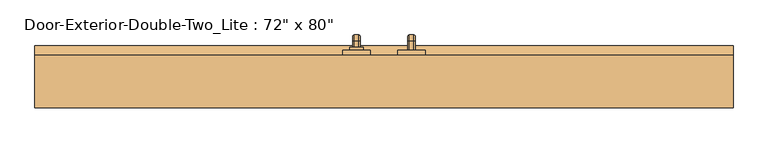
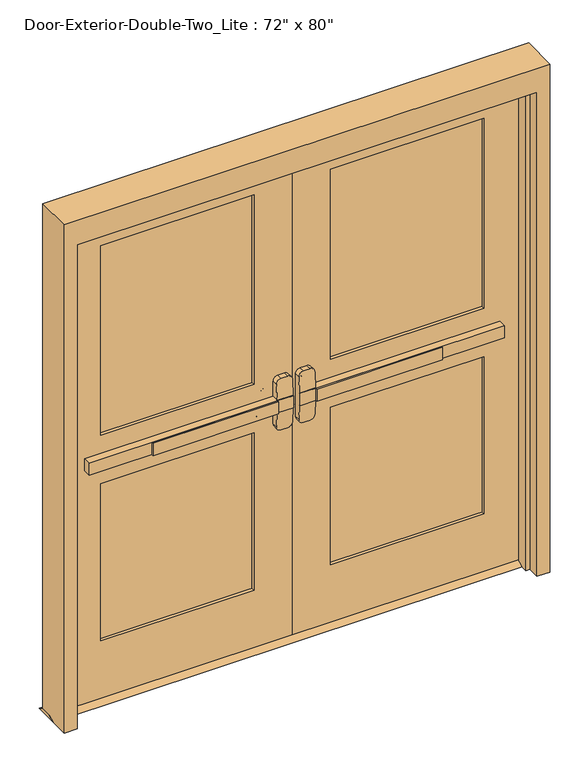
"""IFC4 building model written with IfcOpenShell, lengths in millimetres: door geometry."""

from ifc_helpers import new_model, si_unit, point, frame, frame_2d, origin, place, context, project, spatial, polyline, circle_curve, ellipse_curve, trimmed, segment, composite_curve, outline, extrude, faceted_brep, source, transform, mapped, element, save
from ifc_brep_helpers import plane_surface, cylinder_surface, revolved_surface, advanced_brep


def door_7ac9a1dc(model_context):
    return source(origin(), model_context, "Body", "SolidModel", [
        extrude(outline(polyline([(-575.7333333, -3.175), (-575.7333333, 3.175), (-76.2, 3.175), (-76.2, -3.175), (-575.7333333, -3.175)])), frame((0.0, 0.0, 990.6), z_axis=(0.0, 0.0, 1.0), x_axis=(1.0, 0.0, 0.0)), (0.0, 0.0, 1.0), 50.8),
        advanced_brep(
        [(-12.7, 3.175, 1041.4), (-76.2, 3.175, 1041.4), (-825.5, 3.175, 1041.4), (-825.5, 3.175, 990.6), (-76.2, 3.175, 990.6), (-12.7, 3.175, 990.6), (-825.5, 34.925, 1041.4), (-76.2, 34.925, 1041.4), (-76.2, 34.925, 1104.9), (-57.15, 34.925, 1123.95), (-31.75, 34.925, 1123.95), (-12.7, 34.925, 1104.9), (-12.7, 34.925, 927.1), (-31.75, 34.925, 908.05), (-57.15, 34.925, 908.05), (-76.2, 34.925, 927.1), (-76.2, 34.925, 990.6), (-825.5, 34.925, 990.6), (-12.7, 6.3502467, 1041.4), (-76.2, 6.3502467, 1041.4), (-12.7, 6.3502467, 990.6), (-12.7, 11.3604269, 927.1), (-12.7, 11.3604269, 1104.9), (-76.2, 6.3502467, 990.6), (-76.2, 11.3604269, 1104.9), (-76.2, 11.3604269, 927.1), (-57.15, 12.863481, 1123.95), (-31.75, 12.863481, 1123.95), (-31.75, 12.863481, 908.05), (-57.15, 12.863481, 908.05)],
        [
            (0, 1),
            (1, 2),
            (2, 3),
            (3, 4),
            (4, 5),
            (5, 0),
            (6, 7),
            (7, 8),
            (8, 9, circle_curve(frame((-57.15, 34.925, 1104.9), z_axis=(0.0, 1.0, 0.0), x_axis=(-1.0, 0.0, 0.0)), 19.05)),
            (9, 10),
            (10, 11, circle_curve(frame((-31.75, 34.925, 1104.9), z_axis=(0.0, 1.0, 0.0), x_axis=(-1.0, 0.0, 0.0)), 19.05)),
            (11, 12),
            (12, 13, circle_curve(frame((-31.75, 34.925, 927.1), z_axis=(0.0, 1.0, 0.0), x_axis=(-1.0, 0.0, 0.0)), 19.05)),
            (13, 14),
            (14, 15, circle_curve(frame((-57.15, 34.925, 927.1), z_axis=(0.0, 1.0, 0.0), x_axis=(-1.0, 0.0, 0.0)), 19.05)),
            (15, 16),
            (16, 17),
            (17, 6),
            (0, 18),
            (18, 19),
            (19, 7),
            (6, 2),
            (5, 20),
            (20, 21),
            (21, 12),
            (11, 22),
            (22, 18),
            (16, 23),
            (23, 20),
            (3, 17),
            (19, 24),
            (24, 8),
            (15, 25),
            (25, 23),
            (9, 26),
            (26, 27),
            (27, 10),
            (13, 28),
            (28, 29),
            (29, 14),
            (29, 25, ellipse_curve(frame((-57.15, 11.3604269, 927.1), z_axis=(0.0, 0.9969018152893365, 0.07865602756830282), x_axis=(0.0, -0.07865602756830208, 0.9969018152893365)), 19.1092038, 19.05)),
            (24, 26, ellipse_curve(frame((-57.15, 11.3604269, 1104.9), z_axis=(0.0, 0.9969018152893376, -0.07865602756828934), x_axis=(0.0, -0.078656027568288, -0.9969018152893377)), 19.1092038, 19.05)),
            (27, 22, ellipse_curve(frame((-31.75, 11.3604269, 1104.9), z_axis=(0.0, 0.9969018152893376, -0.07865602756828934), x_axis=(0.0, -0.078656027568288, -0.9969018152893377)), 19.1092038, 19.05)),
            (21, 28, ellipse_curve(frame((-31.75, 11.3604269, 927.1), z_axis=(0.0, 0.9969018152893365, 0.07865602756830282), x_axis=(0.0, -0.07865602756830208, 0.9969018152893365)), 19.1092038, 19.05)),
        ],
        [
            plane_surface(frame((-12.7, 3.175, 1041.4), z_axis=(0.0, -1.0, 0.0), x_axis=(1.0, 0.0, 0.0))),
            plane_surface(frame((-12.7, 34.925, 1041.4), z_axis=(0.0, 1.0, 0.0), x_axis=(-1.0, 0.0, 0.0))),
            plane_surface(frame((-825.5, 3.175, 1041.4), z_axis=(0.0, 0.0, 1.0), x_axis=(0.0, 1.0, 0.0))),
            plane_surface(frame((-12.7, 3.175, 1041.4), z_axis=(1.0, 0.0, 0.0), x_axis=(0.0, 1.0, 0.0))),
            plane_surface(frame((-12.7, 3.175, 990.6), z_axis=(0.0, 0.0, -1.0), x_axis=(0.0, 1.0, 0.0))),
            plane_surface(frame((-825.5, 3.175, 990.6), z_axis=(-1.0, 0.0, 0.0), x_axis=(0.0, 1.0, 0.0))),
            plane_surface(frame((-76.2, 6.3502467, 927.1), z_axis=(-1.0, 0.0, 0.0), x_axis=(0.0, 1.0, 0.0))),
            plane_surface(frame((-57.15, 6.3502467, 1123.95), z_axis=(0.0, 0.0, 1.0), x_axis=(0.0, 1.0, 0.0))),
            plane_surface(frame((-31.75, 6.3502467, 908.05), z_axis=(0.0, 0.0, -1.0), x_axis=(0.0, 1.0, 0.0))),
            cylinder_surface(frame((-57.15, 34.925, 927.1), z_axis=(0.0, -1.0, 0.0), x_axis=(-1.0, 0.0, 0.0)), 19.05),
            cylinder_surface(frame((-57.15, 34.925, 1104.9), z_axis=(0.0, -1.0, 0.0), x_axis=(-1.0, 0.0, 0.0)), 19.05),
            cylinder_surface(frame((-31.75, 34.925, 1104.9), z_axis=(0.0, -1.0, 0.0), x_axis=(-1.0, 0.0, 0.0)), 19.05),
            cylinder_surface(frame((-31.75, 34.925, 927.1), z_axis=(0.0, -1.0, 0.0), x_axis=(-1.0, 0.0, 0.0)), 19.05),
            plane_surface(frame((-76.2, 6.3502467, 1041.4), z_axis=(0.0, -0.9969018152893376, 0.07865602756828934), x_axis=(1.0, 0.0, 0.0))),
            plane_surface(frame((-76.2, 12.863481, 908.05), z_axis=(0.0, -0.9969018152893365, -0.07865602756830282), x_axis=(1.0, 0.0, 0.0))),
        ],
        [
            (0, [[1, 2, 3, 4, 5, 6]]),
            (1, [[7, 8, 9, 10, 11, 12, 13, 14, 15, 16, 17, 18]]),
            (2, [[-2, -1, 19, 20, 21, -7, 22]]),
            (3, [[23, 24, 25, -12, 26, 27, -19, -6]]),
            (4, [[-17, 28, 29, -23, -5, -4, 30]]),
            (5, [[-22, -18, -30, -3]]),
            (6, [[-21, 31, 32, -8]]),
            (6, [[33, 34, -28, -16]]),
            (7, [[35, 36, 37, -10]]),
            (8, [[38, 39, 40, -14]]),
            (9, [[-40, 41, -33, -15]]),
            (10, [[-32, 42, -35, -9]]),
            (11, [[-37, 43, -26, -11]]),
            (12, [[-25, 44, -38, -13]]),
            (13, [[-27, -43, -36, -42, -31, -20]]),
            (14, [[-29, -34, -41, -39, -44, -24]]),
        ],
    ),
        extrude(outline(polyline([(79.375, 12.7), (104.775, 0.0), (9.525, 0.0), (34.925, 12.7), (79.375, 12.7)])), frame((-965.2, 0.0, 0.0), z_axis=(1.0, 0.0, 0.0), x_axis=(0.0, 1.0, 0.0)), (0.0, 0.0, 1.0), 1930.4),
        extrude(outline(polyline([(575.7333333, -3.175), (76.2, -3.175), (76.2, 3.175), (575.7333333, 3.175), (575.7333333, -3.175)])), frame((0.0, 0.0, 990.6), z_axis=(0.0, 0.0, 1.0), x_axis=(1.0, 0.0, 0.0)), (0.0, 0.0, 1.0), 50.8),
        advanced_brep(
        [(12.7, 3.175, 1041.4), (12.7, 3.175, 990.6), (76.2, 3.175, 990.6), (825.5, 3.175, 990.6), (825.5, 3.175, 1041.4), (76.2, 3.175, 1041.4), (825.5, 34.925, 1041.4), (825.5, 34.925, 990.6), (76.2, 34.925, 990.6), (76.2, 34.925, 927.1), (57.15, 34.925, 908.05), (31.75, 34.925, 908.05), (12.7, 34.925, 927.1), (12.7, 34.925, 1104.9), (31.75, 34.925, 1123.95), (57.15, 34.925, 1123.95), (76.2, 34.925, 1104.9), (76.2, 34.925, 1041.4), (76.2, 6.3502467, 1041.4), (12.7, 6.3502467, 1041.4), (12.7, 11.3604269, 1104.9), (12.7, 11.3604269, 927.1), (12.7, 6.3502467, 990.6), (76.2, 6.3502467, 990.6), (76.2, 11.3604269, 927.1), (76.2, 11.3604269, 1104.9), (31.75, 12.863481, 1123.95), (57.15, 12.863481, 1123.95), (57.15, 12.863481, 908.05), (31.75, 12.863481, 908.05)],
        [
            (0, 1),
            (1, 2),
            (2, 3),
            (3, 4),
            (4, 5),
            (5, 0),
            (6, 7),
            (7, 8),
            (8, 9),
            (9, 10, circle_curve(frame((57.15, 34.925, 927.1), z_axis=(0.0, 1.0, 0.0), x_axis=(1.0, 0.0, 0.0)), 19.05)),
            (10, 11),
            (11, 12, circle_curve(frame((31.75, 34.925, 927.1), z_axis=(0.0, 1.0, 0.0), x_axis=(1.0, 0.0, 0.0)), 19.05)),
            (12, 13),
            (13, 14, circle_curve(frame((31.75, 34.925, 1104.9), z_axis=(0.0, 1.0, 0.0), x_axis=(1.0, 0.0, 0.0)), 19.05)),
            (14, 15),
            (15, 16, circle_curve(frame((57.15, 34.925, 1104.9), z_axis=(0.0, 1.0, 0.0), x_axis=(1.0, 0.0, 0.0)), 19.05)),
            (16, 17),
            (17, 6),
            (4, 6),
            (17, 18),
            (18, 19),
            (19, 0),
            (19, 20),
            (20, 13),
            (12, 21),
            (21, 22),
            (22, 1),
            (7, 3),
            (22, 23),
            (23, 8),
            (23, 24),
            (24, 9),
            (16, 25),
            (25, 18),
            (14, 26),
            (26, 27),
            (27, 15),
            (10, 28),
            (28, 29),
            (29, 11),
            (24, 28, ellipse_curve(frame((57.15, 11.3604269, 927.1), z_axis=(0.0, 0.9969018152893365, 0.07865602756830282), x_axis=(0.0, -0.07865602756830208, 0.9969018152893365)), 19.1092038, 19.05)),
            (27, 25, ellipse_curve(frame((57.15, 11.3604269, 1104.9), z_axis=(0.0, 0.9969018152893376, -0.07865602756828934), x_axis=(0.0, -0.078656027568288, -0.9969018152893377)), 19.1092038, 19.05)),
            (20, 26, ellipse_curve(frame((31.75, 11.3604269, 1104.9), z_axis=(0.0, 0.9969018152893376, -0.07865602756828934), x_axis=(0.0, -0.078656027568288, -0.9969018152893377)), 19.1092038, 19.05)),
            (29, 21, ellipse_curve(frame((31.75, 11.3604269, 927.1), z_axis=(0.0, 0.9969018152893365, 0.07865602756830282), x_axis=(0.0, -0.07865602756830208, 0.9969018152893365)), 19.1092038, 19.05)),
        ],
        [
            plane_surface(frame((12.7, 3.175, 1041.4), z_axis=(0.0, -1.0, 0.0), x_axis=(-1.0, 0.0, 0.0))),
            plane_surface(frame((12.7, 34.925, 1041.4), z_axis=(0.0, 1.0, 0.0), x_axis=(1.0, 0.0, 0.0))),
            plane_surface(frame((825.5, 3.175, 1041.4), z_axis=(0.0, 0.0, 1.0), x_axis=(0.0, 1.0, 0.0))),
            plane_surface(frame((12.7, 3.175, 1041.4), z_axis=(-1.0, 0.0, 0.0), x_axis=(0.0, 1.0, 0.0))),
            plane_surface(frame((12.7, 3.175, 990.6), z_axis=(0.0, 0.0, -1.0), x_axis=(0.0, 1.0, 0.0))),
            plane_surface(frame((825.5, 3.175, 990.6), z_axis=(1.0, 0.0, 0.0), x_axis=(0.0, 1.0, 0.0))),
            plane_surface(frame((76.2, 6.3502467, 927.1), z_axis=(1.0, 0.0, 0.0), x_axis=(0.0, 1.0, 0.0))),
            plane_surface(frame((57.15, 6.3502467, 1123.95), z_axis=(0.0, 0.0, 1.0), x_axis=(0.0, 1.0, 0.0))),
            plane_surface(frame((31.75, 6.3502467, 908.05), z_axis=(0.0, 0.0, -1.0), x_axis=(0.0, 1.0, 0.0))),
            cylinder_surface(frame((57.15, 34.925, 927.1), z_axis=(0.0, -1.0, 0.0), x_axis=(1.0, 0.0, 0.0)), 19.05),
            cylinder_surface(frame((57.15, 34.925, 1104.9), z_axis=(0.0, -1.0, 0.0), x_axis=(1.0, 0.0, 0.0)), 19.05),
            cylinder_surface(frame((31.75, 34.925, 1104.9), z_axis=(0.0, -1.0, 0.0), x_axis=(1.0, 0.0, 0.0)), 19.05),
            cylinder_surface(frame((31.75, 34.925, 927.1), z_axis=(0.0, -1.0, 0.0), x_axis=(1.0, 0.0, 0.0)), 19.05),
            plane_surface(frame((76.2, 6.3502467, 1041.4), z_axis=(0.0, -0.9969018152893376, 0.07865602756828934), x_axis=(-1.0, 0.0, 0.0))),
            plane_surface(frame((76.2, 12.863481, 908.05), z_axis=(0.0, -0.9969018152893365, -0.07865602756830282), x_axis=(-1.0, 0.0, 0.0))),
        ],
        [
            (0, [[1, 2, 3, 4, 5, 6]]),
            (1, [[7, 8, 9, 10, 11, 12, 13, 14, 15, 16, 17, 18]]),
            (2, [[19, -18, 20, 21, 22, -6, -5]]),
            (3, [[-1, -22, 23, 24, -13, 25, 26, 27]]),
            (4, [[28, -3, -2, -27, 29, 30, -8]]),
            (5, [[-4, -28, -7, -19]]),
            (6, [[-9, -30, 31, 32]]),
            (6, [[-17, 33, 34, -20]]),
            (7, [[-15, 35, 36, 37]]),
            (8, [[-11, 38, 39, 40]]),
            (9, [[-10, -32, 41, -38]]),
            (10, [[-16, -37, 42, -33]]),
            (11, [[-14, -24, 43, -35]]),
            (12, [[-12, -40, 44, -25]]),
            (13, [[-21, -34, -42, -36, -43, -23]]),
            (14, [[-26, -44, -39, -41, -31, -29]]),
        ],
    ),
        advanced_brep(
        [(66.2, 92.075, 1017.190625), (66.2, 92.075, 1014.809375), (69.771875, 92.075, 1011.2375), (82.6284594, 92.075, 1011.2375), (86.2, 92.075, 1014.8090406), (86.2, 92.075, 1017.190625), (82.628125, 92.075, 1020.7625), (69.771875, 92.075, 1020.7625), (66.2, 92.075, 887.809375), (69.771875, 92.075, 884.2375), (82.628125, 92.075, 884.2375), (86.2, 92.075, 887.809375), (86.2, 92.075, 890.1909594), (82.6284594, 92.075, 893.7625), (69.771875, 92.075, 893.7625), (66.2, 92.075, 890.190625), (66.2, 117.475, 1017.190625), (66.2, 131.365625, 1003.3), (66.2, 131.365625, 901.7), (66.2, 117.475, 887.809375), (66.2, 117.475, 890.190625), (66.2, 128.984375, 901.7), (66.2, 128.984375, 1003.3), (66.2, 117.475, 1014.809375), (69.771875, 117.475, 1011.2375), (82.6284594, 117.475, 1011.2375), (86.2, 117.475, 1014.8090406), (86.2, 128.9840406, 1003.3), (86.2, 128.9840406, 901.7), (86.2, 117.475, 890.1909594), (86.2, 117.475, 887.809375), (86.2, 131.365625, 901.7), (86.2, 131.365625, 1003.3), (86.2, 117.475, 1017.190625), (82.628125, 117.475, 1020.7625), (69.771875, 117.475, 1020.7625), (69.771875, 125.4125, 1003.3), (82.6284594, 125.4125, 1003.3), (82.628125, 134.9375, 1003.3), (69.771875, 134.9375, 1003.3), (69.771875, 125.4125, 901.7), (82.6284594, 125.4125, 901.7), (82.628125, 134.9375, 901.7), (69.771875, 134.9375, 901.7), (69.771875, 117.475, 893.7625), (82.6284594, 117.475, 893.7625), (82.628125, 117.475, 884.2375), (69.771875, 117.475, 884.2375)],
        [
            (0, 1),
            (1, 2, circle_curve(frame((69.771875, 92.075, 1014.809375), z_axis=(0.0, -1.0, 0.0), x_axis=(0.0, 0.0, 1.0)), 3.571875)),
            (2, 3),
            (3, 4, circle_curve(frame((82.6284594, 92.075, 1014.8090406), z_axis=(0.0, -1.0, 0.0), x_axis=(0.0, 0.0, 1.0)), 3.5715406)),
            (4, 5),
            (5, 6, circle_curve(frame((82.628125, 92.075, 1017.190625), z_axis=(0.0, -1.0, 0.0), x_axis=(0.0, 0.0, 1.0)), 3.571875)),
            (6, 7),
            (7, 0, circle_curve(frame((69.771875, 92.075, 1017.190625), z_axis=(0.0, -1.0, 0.0), x_axis=(0.0, 0.0, 1.0)), 3.571875)),
            (8, 9, circle_curve(frame((69.771875, 92.075, 887.809375), z_axis=(0.0, -1.0, 0.0), x_axis=(0.0, 0.0, -1.0)), 3.571875)),
            (9, 10),
            (10, 11, circle_curve(frame((82.628125, 92.075, 887.809375), z_axis=(0.0, -1.0, 0.0), x_axis=(0.0, 0.0, -1.0)), 3.571875)),
            (11, 12),
            (12, 13, circle_curve(frame((82.6284594, 92.075, 890.1909594), z_axis=(0.0, -1.0, 0.0), x_axis=(0.0, 0.0, -1.0)), 3.5715406)),
            (13, 14),
            (14, 15, circle_curve(frame((69.771875, 92.075, 890.190625), z_axis=(0.0, -1.0, 0.0), x_axis=(0.0, 0.0, -1.0)), 3.571875)),
            (15, 8),
            (0, 16),
            (16, 17, circle_curve(frame((66.2, 117.475, 1003.3), z_axis=(-1.0, 0.0, 0.0), x_axis=(0.0, 0.0, 1.0)), 13.890625)),
            (17, 18),
            (18, 19, circle_curve(frame((66.2, 117.475, 901.7), z_axis=(-1.0, 0.0, 0.0), x_axis=(0.0, 1.0, 0.0)), 13.890625)),
            (19, 8),
            (15, 20),
            (20, 21, circle_curve(frame((66.2, 117.475, 901.7), z_axis=(1.0, 0.0, 0.0), x_axis=(0.0, 1.0, 0.0)), 11.509375)),
            (21, 22),
            (22, 23, circle_curve(frame((66.2, 117.475, 1003.3), z_axis=(1.0, 0.0, 0.0), x_axis=(0.0, 0.0, 1.0)), 11.509375)),
            (23, 1),
            (23, 24, circle_curve(frame((69.771875, 117.475, 1014.809375), z_axis=(0.0, -1.0, 0.0), x_axis=(0.0, 0.0, 1.0)), 3.571875)),
            (24, 2),
            (24, 25),
            (25, 3),
            (25, 26, circle_curve(frame((82.6284594, 117.475, 1014.8090406), z_axis=(0.0, -1.0, 0.0), x_axis=(0.0, 0.0, 1.0)), 3.5715406)),
            (26, 4),
            (26, 27, circle_curve(frame((86.2, 117.475, 1003.3), z_axis=(-1.0, 0.0, 0.0), x_axis=(0.0, 0.0, 1.0)), 11.5090406)),
            (27, 28),
            (28, 29, circle_curve(frame((86.2, 117.475, 901.7), z_axis=(-1.0, 0.0, 0.0), x_axis=(0.0, 1.0, 0.0)), 11.5090406)),
            (29, 12),
            (11, 30),
            (30, 31, circle_curve(frame((86.2, 117.475, 901.7), z_axis=(1.0, 0.0, 0.0), x_axis=(0.0, 1.0, 0.0)), 13.890625)),
            (31, 32),
            (32, 33, circle_curve(frame((86.2, 117.475, 1003.3), z_axis=(1.0, 0.0, 0.0), x_axis=(0.0, 0.0, 1.0)), 13.890625)),
            (33, 5),
            (33, 34, circle_curve(frame((82.628125, 117.475, 1017.190625), z_axis=(0.0, -1.0, 0.0), x_axis=(0.0, 0.0, 1.0)), 3.571875)),
            (34, 6),
            (34, 35),
            (35, 7),
            (35, 16, circle_curve(frame((69.771875, 117.475, 1017.190625), z_axis=(0.0, -1.0, 0.0), x_axis=(0.0, 0.0, 1.0)), 3.571875)),
            (36, 24, circle_curve(frame((69.771875, 117.475, 1003.3), z_axis=(1.0, 0.0, 0.0), x_axis=(0.0, 0.0, 1.0)), 7.9375)),
            (22, 36, circle_curve(frame((69.771875, 128.984375, 1003.3), z_axis=(0.0, 0.0, 1.0), x_axis=(0.0, 1.0, 0.0)), 3.571875)),
            (37, 25, circle_curve(frame((82.6284594, 117.475, 1003.3), z_axis=(1.0, 0.0, 0.0), x_axis=(0.0, 0.0, 1.0)), 7.9375)),
            (36, 37),
            (37, 27, circle_curve(frame((82.6284594, 128.9840406, 1003.3), z_axis=(0.0, 0.0, 1.0), x_axis=(0.0, 1.0, 0.0)), 3.5715406)),
            (38, 34, circle_curve(frame((82.628125, 117.475, 1003.3), z_axis=(1.0, 0.0, 0.0), x_axis=(0.0, 0.0, 1.0)), 17.4625)),
            (32, 38, circle_curve(frame((82.628125, 131.365625, 1003.3), z_axis=(0.0, 0.0, 1.0), x_axis=(0.0, 1.0, 0.0)), 3.571875)),
            (39, 35, circle_curve(frame((69.771875, 117.475, 1003.3), z_axis=(1.0, 0.0, 0.0), x_axis=(0.0, 0.0, 1.0)), 17.4625)),
            (38, 39),
            (39, 17, circle_curve(frame((69.771875, 131.365625, 1003.3), z_axis=(0.0, 0.0, 1.0), x_axis=(0.0, 1.0, 0.0)), 3.571875)),
            (21, 40, circle_curve(frame((69.771875, 128.984375, 901.7), z_axis=(0.0, 0.0, 1.0), x_axis=(0.0, 1.0, 0.0)), 3.571875)),
            (40, 36),
            (40, 41),
            (41, 37),
            (41, 28, circle_curve(frame((82.6284594, 128.9840406, 901.7), z_axis=(0.0, 0.0, 1.0), x_axis=(0.0, 1.0, 0.0)), 3.5715406)),
            (31, 42, circle_curve(frame((82.628125, 131.365625, 901.7), z_axis=(0.0, 0.0, 1.0), x_axis=(0.0, 1.0, 0.0)), 3.571875)),
            (42, 38),
            (42, 43),
            (43, 39),
            (43, 18, circle_curve(frame((69.771875, 131.365625, 901.7), z_axis=(0.0, 0.0, 1.0), x_axis=(0.0, 1.0, 0.0)), 3.571875)),
            (44, 40, circle_curve(frame((69.771875, 117.475, 901.7), z_axis=(1.0, 0.0, 0.0), x_axis=(0.0, 1.0, 0.0)), 7.9375)),
            (20, 44, circle_curve(frame((69.771875, 117.475, 890.190625), z_axis=(0.0, 1.0, 0.0), x_axis=(0.0, 0.0, -1.0)), 3.571875)),
            (45, 41, circle_curve(frame((82.6284594, 117.475, 901.7), z_axis=(1.0, 0.0, 0.0), x_axis=(0.0, 1.0, 0.0)), 7.9375)),
            (44, 45),
            (45, 29, circle_curve(frame((82.6284594, 117.475, 890.1909594), z_axis=(0.0, 1.0, 0.0), x_axis=(0.0, 0.0, -1.0)), 3.5715406)),
            (46, 42, circle_curve(frame((82.628125, 117.475, 901.7), z_axis=(1.0, 0.0, 0.0), x_axis=(0.0, 1.0, 0.0)), 17.4625)),
            (30, 46, circle_curve(frame((82.628125, 117.475, 887.809375), z_axis=(0.0, 1.0, 0.0), x_axis=(0.0, 0.0, -1.0)), 3.571875)),
            (47, 43, circle_curve(frame((69.771875, 117.475, 901.7), z_axis=(1.0, 0.0, 0.0), x_axis=(0.0, 1.0, 0.0)), 17.4625)),
            (46, 47),
            (47, 19, circle_curve(frame((69.771875, 117.475, 887.809375), z_axis=(0.0, 1.0, 0.0), x_axis=(0.0, 0.0, -1.0)), 3.571875)),
            (14, 44),
            (13, 45),
            (10, 46),
            (9, 47),
        ],
        [
            plane_surface(frame((76.2, 92.075, 1016.0), z_axis=(0.0, -1.0, 0.0), x_axis=(1.0, 0.0, 0.0))),
            plane_surface(frame((76.2, 92.075, 889.0), z_axis=(0.0, -1.0, 0.0), x_axis=(1.0, 0.0, 0.0))),
            plane_surface(frame((66.2, 92.075, 1017.190625), z_axis=(-1.0, 0.0, 0.0), x_axis=(0.0, 1.0, 0.0))),
            cylinder_surface(frame((69.771875, 92.075, 1014.809375), z_axis=(0.0, -1.0, 0.0), x_axis=(0.0, 0.0, 1.0)), 3.571875),
            plane_surface(frame((69.771875, 92.075, 1011.2375), z_axis=(0.0, 0.0, -1.0), x_axis=(0.0, 1.0, 0.0))),
            cylinder_surface(frame((82.6284594, 92.075, 1014.8090406), z_axis=(0.0, -1.0, 0.0), x_axis=(0.0, 0.0, 1.0)), 3.5715406),
            plane_surface(frame((86.2, 92.075, 1014.8090406), z_axis=(1.0, 0.0, 0.0), x_axis=(0.0, 1.0, 0.0))),
            cylinder_surface(frame((82.628125, 92.075, 1017.190625), z_axis=(0.0, -1.0, 0.0), x_axis=(0.0, 0.0, 1.0)), 3.571875),
            plane_surface(frame((82.628125, 92.075, 1020.7625), z_axis=(0.0, 0.0, 1.0), x_axis=(0.0, 1.0, 0.0))),
            cylinder_surface(frame((69.771875, 92.075, 1017.190625), z_axis=(0.0, -1.0, 0.0), x_axis=(0.0, 0.0, 1.0)), 3.571875),
            revolved_surface(trimmed(ellipse_curve(frame((69.771875, 117.475, 1014.809375), z_axis=(0.0, -1.0, 0.0), x_axis=(0.0, 0.0, 1.0)), 3.571875, 3.571875), [point((66.2, 117.475, 1014.809375))], [point((69.771875, 117.475, 1011.2375))], True, "CARTESIAN"), (76.2, 117.475, 1003.3), (-1.0, 0.0, 0.0)),
            revolved_surface(polyline([(69.771875, 117.475, 1011.2375), (82.6284594, 117.475, 1011.2375)]), (76.2, 117.475, 1003.3), (-1.0, 0.0, 0.0)),
            revolved_surface(trimmed(ellipse_curve(frame((82.6284594, 117.475, 1014.8090406), z_axis=(0.0, -1.0, 0.0), x_axis=(0.0, 0.0, 1.0)), 3.5715406, 3.5715406), [point((82.6284594, 117.475, 1011.2375))], [point((86.2, 117.475, 1014.8090406))], True, "CARTESIAN"), (76.2, 117.475, 1003.3), (-1.0, 0.0, 0.0)),
            revolved_surface(trimmed(ellipse_curve(frame((82.628125, 117.475, 1017.190625), z_axis=(0.0, -1.0, 0.0), x_axis=(0.0, 0.0, 1.0)), 3.571875, 3.571875), [point((86.2, 117.475, 1017.190625))], [point((82.628125, 117.475, 1020.7625))], True, "CARTESIAN"), (76.2, 117.475, 1003.3), (-1.0, 0.0, 0.0)),
            cylinder_surface(frame((76.2, 117.475, 1003.3), z_axis=(-1.0, 0.0, 0.0), x_axis=(0.0, 0.0, 1.0)), 17.4625),
            revolved_surface(trimmed(ellipse_curve(frame((69.771875, 117.475, 1017.190625), z_axis=(0.0, -1.0, 0.0), x_axis=(0.0, 0.0, 1.0)), 3.571875, 3.571875), [point((69.771875, 117.475, 1020.7625))], [point((66.2, 117.475, 1017.190625))], True, "CARTESIAN"), (76.2, 117.475, 1003.3), (-1.0, 0.0, 0.0)),
            cylinder_surface(frame((69.771875, 128.984375, 1003.3), z_axis=(0.0, 0.0, 1.0), x_axis=(0.0, 1.0, 0.0)), 3.571875),
            plane_surface(frame((69.771875, 125.4125, 1003.3), z_axis=(0.0, -1.0, 0.0), x_axis=(0.0, 0.0, -1.0))),
            cylinder_surface(frame((82.6284594, 128.9840406, 1003.3), z_axis=(0.0, 0.0, 1.0), x_axis=(0.0, 1.0, 0.0)), 3.5715406),
            cylinder_surface(frame((82.628125, 131.365625, 1003.3), z_axis=(0.0, 0.0, 1.0), x_axis=(0.0, 1.0, 0.0)), 3.571875),
            plane_surface(frame((82.628125, 134.9375, 1003.3), z_axis=(0.0, 1.0, 0.0), x_axis=(0.0, 0.0, -1.0))),
            cylinder_surface(frame((69.771875, 131.365625, 1003.3), z_axis=(0.0, 0.0, 1.0), x_axis=(0.0, 1.0, 0.0)), 3.571875),
            revolved_surface(trimmed(ellipse_curve(frame((69.771875, 128.984375, 901.7), z_axis=(0.0, 0.0, 1.0), x_axis=(0.0, 1.0, 0.0)), 3.571875, 3.571875), [point((66.2, 128.984375, 901.7))], [point((69.771875, 125.4125, 901.7))], True, "CARTESIAN"), (76.2, 117.475, 901.7), (-1.0, 0.0, 0.0)),
            revolved_surface(polyline([(69.771875, 125.4125, 901.7), (82.6284594, 125.4125, 901.7)]), (76.2, 117.475, 901.7), (-1.0, 0.0, 0.0)),
            revolved_surface(trimmed(ellipse_curve(frame((82.6284594, 128.9840406, 901.7), z_axis=(0.0, 0.0, 1.0), x_axis=(0.0, 1.0, 0.0)), 3.5715406, 3.5715406), [point((82.6284594, 125.4125, 901.7))], [point((86.2, 128.9840406, 901.7))], True, "CARTESIAN"), (76.2, 117.475, 901.7), (-1.0, 0.0, 0.0)),
            revolved_surface(trimmed(ellipse_curve(frame((82.628125, 131.365625, 901.7), z_axis=(0.0, 0.0, 1.0), x_axis=(0.0, 1.0, 0.0)), 3.571875, 3.571875), [point((86.2, 131.365625, 901.7))], [point((82.628125, 134.9375, 901.7))], True, "CARTESIAN"), (76.2, 117.475, 901.7), (-1.0, 0.0, 0.0)),
            cylinder_surface(frame((76.2, 117.475, 901.7), z_axis=(-1.0, 0.0, 0.0), x_axis=(0.0, 1.0, 0.0)), 17.4625),
            revolved_surface(trimmed(ellipse_curve(frame((69.771875, 131.365625, 901.7), z_axis=(0.0, 0.0, 1.0), x_axis=(0.0, 1.0, 0.0)), 3.571875, 3.571875), [point((69.771875, 134.9375, 901.7))], [point((66.2, 131.365625, 901.7))], True, "CARTESIAN"), (76.2, 117.475, 901.7), (-1.0, 0.0, 0.0)),
            cylinder_surface(frame((69.771875, 117.475, 890.190625), z_axis=(0.0, 1.0, 0.0), x_axis=(0.0, 0.0, -1.0)), 3.571875),
            plane_surface(frame((69.771875, 117.475, 893.7625), z_axis=(0.0, 0.0, 1.0), x_axis=(0.0, -1.0, 0.0))),
            cylinder_surface(frame((82.6284594, 117.475, 890.1909594), z_axis=(0.0, 1.0, 0.0), x_axis=(0.0, 0.0, -1.0)), 3.5715406),
            cylinder_surface(frame((82.628125, 117.475, 887.809375), z_axis=(0.0, 1.0, 0.0), x_axis=(0.0, 0.0, -1.0)), 3.571875),
            plane_surface(frame((82.628125, 117.475, 884.2375), z_axis=(0.0, 0.0, -1.0), x_axis=(0.0, -1.0, 0.0))),
            cylinder_surface(frame((69.771875, 117.475, 887.809375), z_axis=(0.0, 1.0, 0.0), x_axis=(0.0, 0.0, -1.0)), 3.571875),
        ],
        [
            (0, [[1, 2, 3, 4, 5, 6, 7, 8]]),
            (1, [[9, 10, 11, 12, 13, 14, 15, 16]]),
            (2, [[-1, 17, 18, 19, 20, 21, -16, 22, 23, 24, 25, 26]]),
            (3, [[-2, -26, 27, 28]]),
            (4, [[-3, -28, 29, 30]]),
            (5, [[-4, -30, 31, 32]]),
            (6, [[-5, -32, 33, 34, 35, 36, -12, 37, 38, 39, 40, 41]]),
            (7, [[-6, -41, 42, 43]]),
            (8, [[-7, -43, 44, 45]]),
            (9, [[-8, -45, 46, -17]]),
            (10, [[47, -27, -25, 48]]),
            (11, [[49, -29, -47, 50]]),
            (12, [[-33, -31, -49, 51]]),
            (13, [[52, -42, -40, 53]]),
            (14, [[54, -44, -52, 55]]),
            (15, [[-18, -46, -54, 56]]),
            (16, [[-48, -24, 57, 58]]),
            (17, [[-50, -58, 59, 60]]),
            (18, [[-51, -60, 61, -34]]),
            (19, [[-53, -39, 62, 63]]),
            (20, [[-55, -63, 64, 65]]),
            (21, [[-56, -65, 66, -19]]),
            (22, [[67, -57, -23, 68]]),
            (23, [[69, -59, -67, 70]]),
            (24, [[-35, -61, -69, 71]]),
            (25, [[72, -62, -38, 73]]),
            (26, [[74, -64, -72, 75]]),
            (27, [[-20, -66, -74, 76]]),
            (28, [[-68, -22, -15, 77]]),
            (29, [[-70, -77, -14, 78]]),
            (30, [[-71, -78, -13, -36]]),
            (31, [[-73, -37, -11, 79]]),
            (32, [[-75, -79, -10, 80]]),
            (33, [[-76, -80, -9, -21]]),
        ],
    ),
        extrude(outline(composite_curve([segment(trimmed(circle_curve(frame_2d((1113.0338574, 76.2)), 89.3016225), [point((1193.8, 114.3))], [point((1193.8, 38.1))], False, "CARTESIAN"), True, "CONTINUOUS"), segment(polyline([(1193.8, 38.1), (838.2, 38.1)]), True, "CONTINUOUS"), segment(trimmed(circle_curve(frame_2d((918.9661426, 76.2)), 89.3016225), [point((838.2, 38.1))], [point((838.2, 114.3))], False, "CARTESIAN"), True, "CONTINUOUS"), segment(polyline([(838.2, 114.3), (1193.8, 114.3)]), True, "CONTINUOUS")], self_intersect=False)), frame((0.0, 79.375, 0.0), z_axis=(0.0, 1.0, 0.0), x_axis=(0.0, 0.0, 1.0)), (0.0, 0.0, 1.0), 12.7),
        advanced_brep(
        [(-86.2, 92.075, 1017.190625), (-86.2, 92.075, 1014.809375), (-82.628125, 92.075, 1011.2375), (-69.7715406, 92.075, 1011.2375), (-66.2, 92.075, 1014.8090406), (-66.2, 92.075, 1017.190625), (-69.771875, 92.075, 1020.7625), (-82.628125, 92.075, 1020.7625), (-86.2, 92.075, 887.809375), (-82.628125, 92.075, 884.2375), (-69.771875, 92.075, 884.2375), (-66.2, 92.075, 887.809375), (-66.2, 92.075, 890.1909594), (-69.7715406, 92.075, 893.7625), (-82.628125, 92.075, 893.7625), (-86.2, 92.075, 890.190625), (-86.2, 117.475, 1017.190625), (-86.2, 131.365625, 1003.3), (-86.2, 131.365625, 901.7), (-86.2, 117.475, 887.809375), (-86.2, 117.475, 890.190625), (-86.2, 128.984375, 901.7), (-86.2, 128.984375, 1003.3), (-86.2, 117.475, 1014.809375), (-82.628125, 117.475, 1011.2375), (-69.7715406, 117.475, 1011.2375), (-66.2, 117.475, 1014.8090406), (-66.2, 128.9840406, 1003.3), (-66.2, 128.9840406, 901.7), (-66.2, 117.475, 890.1909594), (-66.2, 117.475, 887.809375), (-66.2, 131.365625, 901.7), (-66.2, 131.365625, 1003.3), (-66.2, 117.475, 1017.190625), (-69.771875, 117.475, 1020.7625), (-82.628125, 117.475, 1020.7625), (-82.628125, 125.4125, 1003.3), (-69.7715406, 125.4125, 1003.3), (-69.771875, 134.9375, 1003.3), (-82.628125, 134.9375, 1003.3), (-82.628125, 125.4125, 901.7), (-69.7715406, 125.4125, 901.7), (-69.771875, 134.9375, 901.7), (-82.628125, 134.9375, 901.7), (-82.628125, 117.475, 893.7625), (-69.7715406, 117.475, 893.7625), (-69.771875, 117.475, 884.2375), (-82.628125, 117.475, 884.2375)],
        [
            (0, 1),
            (1, 2, circle_curve(frame((-82.628125, 92.075, 1014.809375), z_axis=(0.0, -1.0, 0.0), x_axis=(0.0, 0.0, 1.0)), 3.571875)),
            (2, 3),
            (3, 4, circle_curve(frame((-69.7715406, 92.075, 1014.8090406), z_axis=(0.0, -1.0, 0.0), x_axis=(0.0, 0.0, 1.0)), 3.5715406)),
            (4, 5),
            (5, 6, circle_curve(frame((-69.771875, 92.075, 1017.190625), z_axis=(0.0, -1.0, 0.0), x_axis=(0.0, 0.0, 1.0)), 3.571875)),
            (6, 7),
            (7, 0, circle_curve(frame((-82.628125, 92.075, 1017.190625), z_axis=(0.0, -1.0, 0.0), x_axis=(0.0, 0.0, 1.0)), 3.571875)),
            (8, 9, circle_curve(frame((-82.628125, 92.075, 887.809375), z_axis=(0.0, -1.0, 0.0), x_axis=(0.0, 0.0, -1.0)), 3.571875)),
            (9, 10),
            (10, 11, circle_curve(frame((-69.771875, 92.075, 887.809375), z_axis=(0.0, -1.0, 0.0), x_axis=(0.0, 0.0, -1.0)), 3.571875)),
            (11, 12),
            (12, 13, circle_curve(frame((-69.7715406, 92.075, 890.1909594), z_axis=(0.0, -1.0, 0.0), x_axis=(0.0, 0.0, -1.0)), 3.5715406)),
            (13, 14),
            (14, 15, circle_curve(frame((-82.628125, 92.075, 890.190625), z_axis=(0.0, -1.0, 0.0), x_axis=(0.0, 0.0, -1.0)), 3.571875)),
            (15, 8),
            (0, 16),
            (16, 17, circle_curve(frame((-86.2, 117.475, 1003.3), z_axis=(-1.0, 0.0, 0.0), x_axis=(0.0, 0.0, 1.0)), 13.890625)),
            (17, 18),
            (18, 19, circle_curve(frame((-86.2, 117.475, 901.7), z_axis=(-1.0, 0.0, 0.0), x_axis=(0.0, 1.0, 0.0)), 13.890625)),
            (19, 8),
            (15, 20),
            (20, 21, circle_curve(frame((-86.2, 117.475, 901.7), z_axis=(1.0, 0.0, 0.0), x_axis=(0.0, 1.0, 0.0)), 11.509375)),
            (21, 22),
            (22, 23, circle_curve(frame((-86.2, 117.475, 1003.3), z_axis=(1.0, 0.0, 0.0), x_axis=(0.0, 0.0, 1.0)), 11.509375)),
            (23, 1),
            (23, 24, circle_curve(frame((-82.628125, 117.475, 1014.809375), z_axis=(0.0, -1.0, 0.0), x_axis=(0.0, 0.0, 1.0)), 3.571875)),
            (24, 2),
            (24, 25),
            (25, 3),
            (25, 26, circle_curve(frame((-69.7715406, 117.475, 1014.8090406), z_axis=(0.0, -1.0, 0.0), x_axis=(0.0, 0.0, 1.0)), 3.5715406)),
            (26, 4),
            (26, 27, circle_curve(frame((-66.2, 117.475, 1003.3), z_axis=(-1.0, 0.0, 0.0), x_axis=(0.0, 0.0, 1.0)), 11.5090406)),
            (27, 28),
            (28, 29, circle_curve(frame((-66.2, 117.475, 901.7), z_axis=(-1.0, 0.0, 0.0), x_axis=(0.0, 1.0, 0.0)), 11.5090406)),
            (29, 12),
            (11, 30),
            (30, 31, circle_curve(frame((-66.2, 117.475, 901.7), z_axis=(1.0, 0.0, 0.0), x_axis=(0.0, 1.0, 0.0)), 13.890625)),
            (31, 32),
            (32, 33, circle_curve(frame((-66.2, 117.475, 1003.3), z_axis=(1.0, 0.0, 0.0), x_axis=(0.0, 0.0, 1.0)), 13.890625)),
            (33, 5),
            (33, 34, circle_curve(frame((-69.771875, 117.475, 1017.190625), z_axis=(0.0, -1.0, 0.0), x_axis=(0.0, 0.0, 1.0)), 3.571875)),
            (34, 6),
            (34, 35),
            (35, 7),
            (35, 16, circle_curve(frame((-82.628125, 117.475, 1017.190625), z_axis=(0.0, -1.0, 0.0), x_axis=(0.0, 0.0, 1.0)), 3.571875)),
            (36, 24, circle_curve(frame((-82.628125, 117.475, 1003.3), z_axis=(1.0, 0.0, 0.0), x_axis=(0.0, 0.0, 1.0)), 7.9375)),
            (22, 36, circle_curve(frame((-82.628125, 128.984375, 1003.3), z_axis=(0.0, 0.0, 1.0), x_axis=(0.0, 1.0, 0.0)), 3.571875)),
            (37, 25, circle_curve(frame((-69.7715406, 117.475, 1003.3), z_axis=(1.0, 0.0, 0.0), x_axis=(0.0, 0.0, 1.0)), 7.9375)),
            (36, 37),
            (37, 27, circle_curve(frame((-69.7715406, 128.9840406, 1003.3), z_axis=(0.0, 0.0, 1.0), x_axis=(0.0, 1.0, 0.0)), 3.5715406)),
            (38, 34, circle_curve(frame((-69.771875, 117.475, 1003.3), z_axis=(1.0, 0.0, 0.0), x_axis=(0.0, 0.0, 1.0)), 17.4625)),
            (32, 38, circle_curve(frame((-69.771875, 131.365625, 1003.3), z_axis=(0.0, 0.0, 1.0), x_axis=(0.0, 1.0, 0.0)), 3.571875)),
            (39, 35, circle_curve(frame((-82.628125, 117.475, 1003.3), z_axis=(1.0, 0.0, 0.0), x_axis=(0.0, 0.0, 1.0)), 17.4625)),
            (38, 39),
            (39, 17, circle_curve(frame((-82.628125, 131.365625, 1003.3), z_axis=(0.0, 0.0, 1.0), x_axis=(0.0, 1.0, 0.0)), 3.571875)),
            (21, 40, circle_curve(frame((-82.628125, 128.984375, 901.7), z_axis=(0.0, 0.0, 1.0), x_axis=(0.0, 1.0, 0.0)), 3.571875)),
            (40, 36),
            (40, 41),
            (41, 37),
            (41, 28, circle_curve(frame((-69.7715406, 128.9840406, 901.7), z_axis=(0.0, 0.0, 1.0), x_axis=(0.0, 1.0, 0.0)), 3.5715406)),
            (31, 42, circle_curve(frame((-69.771875, 131.365625, 901.7), z_axis=(0.0, 0.0, 1.0), x_axis=(0.0, 1.0, 0.0)), 3.571875)),
            (42, 38),
            (42, 43),
            (43, 39),
            (43, 18, circle_curve(frame((-82.628125, 131.365625, 901.7), z_axis=(0.0, 0.0, 1.0), x_axis=(0.0, 1.0, 0.0)), 3.571875)),
            (44, 40, circle_curve(frame((-82.628125, 117.475, 901.7), z_axis=(1.0, 0.0, 0.0), x_axis=(0.0, 1.0, 0.0)), 7.9375)),
            (20, 44, circle_curve(frame((-82.628125, 117.475, 890.190625), z_axis=(0.0, 1.0, 0.0), x_axis=(0.0, 0.0, -1.0)), 3.571875)),
            (45, 41, circle_curve(frame((-69.7715406, 117.475, 901.7), z_axis=(1.0, 0.0, 0.0), x_axis=(0.0, 1.0, 0.0)), 7.9375)),
            (44, 45),
            (45, 29, circle_curve(frame((-69.7715406, 117.475, 890.1909594), z_axis=(0.0, 1.0, 0.0), x_axis=(0.0, 0.0, -1.0)), 3.5715406)),
            (46, 42, circle_curve(frame((-69.771875, 117.475, 901.7), z_axis=(1.0, 0.0, 0.0), x_axis=(0.0, 1.0, 0.0)), 17.4625)),
            (30, 46, circle_curve(frame((-69.771875, 117.475, 887.809375), z_axis=(0.0, 1.0, 0.0), x_axis=(0.0, 0.0, -1.0)), 3.571875)),
            (47, 43, circle_curve(frame((-82.628125, 117.475, 901.7), z_axis=(1.0, 0.0, 0.0), x_axis=(0.0, 1.0, 0.0)), 17.4625)),
            (46, 47),
            (47, 19, circle_curve(frame((-82.628125, 117.475, 887.809375), z_axis=(0.0, 1.0, 0.0), x_axis=(0.0, 0.0, -1.0)), 3.571875)),
            (14, 44),
            (13, 45),
            (10, 46),
            (9, 47),
        ],
        [
            plane_surface(frame((-76.2, 92.075, 1016.0), z_axis=(0.0, -1.0, 0.0), x_axis=(1.0, 0.0, 0.0))),
            plane_surface(frame((-76.2, 92.075, 889.0), z_axis=(0.0, -1.0, 0.0), x_axis=(1.0, 0.0, 0.0))),
            plane_surface(frame((-86.2, 92.075, 1017.190625), z_axis=(-1.0, 0.0, 0.0), x_axis=(0.0, 1.0, 0.0))),
            cylinder_surface(frame((-82.628125, 92.075, 1014.809375), z_axis=(0.0, -1.0, 0.0), x_axis=(0.0, 0.0, 1.0)), 3.571875),
            plane_surface(frame((-82.628125, 92.075, 1011.2375), z_axis=(0.0, 0.0, -1.0), x_axis=(0.0, 1.0, 0.0))),
            cylinder_surface(frame((-69.7715406, 92.075, 1014.8090406), z_axis=(0.0, -1.0, 0.0), x_axis=(0.0, 0.0, 1.0)), 3.5715406),
            plane_surface(frame((-66.2, 92.075, 1014.8090406), z_axis=(1.0, 0.0, 0.0), x_axis=(0.0, 1.0, 0.0))),
            cylinder_surface(frame((-69.771875, 92.075, 1017.190625), z_axis=(0.0, -1.0, 0.0), x_axis=(0.0, 0.0, 1.0)), 3.571875),
            plane_surface(frame((-69.771875, 92.075, 1020.7625), z_axis=(0.0, 0.0, 1.0), x_axis=(0.0, 1.0, 0.0))),
            cylinder_surface(frame((-82.628125, 92.075, 1017.190625), z_axis=(0.0, -1.0, 0.0), x_axis=(0.0, 0.0, 1.0)), 3.571875),
            revolved_surface(trimmed(ellipse_curve(frame((-82.628125, 117.475, 1014.809375), z_axis=(0.0, -1.0, 0.0), x_axis=(0.0, 0.0, 1.0)), 3.571875, 3.571875), [point((-86.2, 117.475, 1014.809375))], [point((-82.628125, 117.475, 1011.2375))], True, "CARTESIAN"), (-76.2, 117.475, 1003.3), (-1.0, 0.0, 0.0)),
            revolved_surface(polyline([(-82.628125, 117.475, 1011.2375), (-69.7715406, 117.475, 1011.2375)]), (-76.2, 117.475, 1003.3), (-1.0, 0.0, 0.0)),
            revolved_surface(trimmed(ellipse_curve(frame((-69.7715406, 117.475, 1014.8090406), z_axis=(0.0, -1.0, 0.0), x_axis=(0.0, 0.0, 1.0)), 3.5715406, 3.5715406), [point((-69.7715406, 117.475, 1011.2375))], [point((-66.2, 117.475, 1014.8090406))], True, "CARTESIAN"), (-76.2, 117.475, 1003.3), (-1.0, 0.0, 0.0)),
            revolved_surface(trimmed(ellipse_curve(frame((-69.771875, 117.475, 1017.190625), z_axis=(0.0, -1.0, 0.0), x_axis=(0.0, 0.0, 1.0)), 3.571875, 3.571875), [point((-66.2, 117.475, 1017.190625))], [point((-69.771875, 117.475, 1020.7625))], True, "CARTESIAN"), (-76.2, 117.475, 1003.3), (-1.0, 0.0, 0.0)),
            cylinder_surface(frame((-76.2, 117.475, 1003.3), z_axis=(-1.0, 0.0, 0.0), x_axis=(0.0, 0.0, 1.0)), 17.4625),
            revolved_surface(trimmed(ellipse_curve(frame((-82.628125, 117.475, 1017.190625), z_axis=(0.0, -1.0, 0.0), x_axis=(0.0, 0.0, 1.0)), 3.571875, 3.571875), [point((-82.628125, 117.475, 1020.7625))], [point((-86.2, 117.475, 1017.190625))], True, "CARTESIAN"), (-76.2, 117.475, 1003.3), (-1.0, 0.0, 0.0)),
            cylinder_surface(frame((-82.628125, 128.984375, 1003.3), z_axis=(0.0, 0.0, 1.0), x_axis=(0.0, 1.0, 0.0)), 3.571875),
            plane_surface(frame((-82.628125, 125.4125, 1003.3), z_axis=(0.0, -1.0, 0.0), x_axis=(0.0, 0.0, -1.0))),
            cylinder_surface(frame((-69.7715406, 128.9840406, 1003.3), z_axis=(0.0, 0.0, 1.0), x_axis=(0.0, 1.0, 0.0)), 3.5715406),
            cylinder_surface(frame((-69.771875, 131.365625, 1003.3), z_axis=(0.0, 0.0, 1.0), x_axis=(0.0, 1.0, 0.0)), 3.571875),
            plane_surface(frame((-69.771875, 134.9375, 1003.3), z_axis=(0.0, 1.0, 0.0), x_axis=(0.0, 0.0, -1.0))),
            cylinder_surface(frame((-82.628125, 131.365625, 1003.3), z_axis=(0.0, 0.0, 1.0), x_axis=(0.0, 1.0, 0.0)), 3.571875),
            revolved_surface(trimmed(ellipse_curve(frame((-82.628125, 128.984375, 901.7), z_axis=(0.0, 0.0, 1.0), x_axis=(0.0, 1.0, 0.0)), 3.571875, 3.571875), [point((-86.2, 128.984375, 901.7))], [point((-82.628125, 125.4125, 901.7))], True, "CARTESIAN"), (-76.2, 117.475, 901.7), (-1.0, 0.0, 0.0)),
            revolved_surface(polyline([(-82.628125, 125.4125, 901.7), (-69.7715406, 125.4125, 901.7)]), (-76.2, 117.475, 901.7), (-1.0, 0.0, 0.0)),
            revolved_surface(trimmed(ellipse_curve(frame((-69.7715406, 128.9840406, 901.7), z_axis=(0.0, 0.0, 1.0), x_axis=(0.0, 1.0, 0.0)), 3.5715406, 3.5715406), [point((-69.7715406, 125.4125, 901.7))], [point((-66.2, 128.9840406, 901.7))], True, "CARTESIAN"), (-76.2, 117.475, 901.7), (-1.0, 0.0, 0.0)),
            revolved_surface(trimmed(ellipse_curve(frame((-69.771875, 131.365625, 901.7), z_axis=(0.0, 0.0, 1.0), x_axis=(0.0, 1.0, 0.0)), 3.571875, 3.571875), [point((-66.2, 131.365625, 901.7))], [point((-69.771875, 134.9375, 901.7))], True, "CARTESIAN"), (-76.2, 117.475, 901.7), (-1.0, 0.0, 0.0)),
            cylinder_surface(frame((-76.2, 117.475, 901.7), z_axis=(-1.0, 0.0, 0.0), x_axis=(0.0, 1.0, 0.0)), 17.4625),
            revolved_surface(trimmed(ellipse_curve(frame((-82.628125, 131.365625, 901.7), z_axis=(0.0, 0.0, 1.0), x_axis=(0.0, 1.0, 0.0)), 3.571875, 3.571875), [point((-82.628125, 134.9375, 901.7))], [point((-86.2, 131.365625, 901.7))], True, "CARTESIAN"), (-76.2, 117.475, 901.7), (-1.0, 0.0, 0.0)),
            cylinder_surface(frame((-82.628125, 117.475, 890.190625), z_axis=(0.0, 1.0, 0.0), x_axis=(0.0, 0.0, -1.0)), 3.571875),
            plane_surface(frame((-82.628125, 117.475, 893.7625), z_axis=(0.0, 0.0, 1.0), x_axis=(0.0, -1.0, 0.0))),
            cylinder_surface(frame((-69.7715406, 117.475, 890.1909594), z_axis=(0.0, 1.0, 0.0), x_axis=(0.0, 0.0, -1.0)), 3.5715406),
            cylinder_surface(frame((-69.771875, 117.475, 887.809375), z_axis=(0.0, 1.0, 0.0), x_axis=(0.0, 0.0, -1.0)), 3.571875),
            plane_surface(frame((-69.771875, 117.475, 884.2375), z_axis=(0.0, 0.0, -1.0), x_axis=(0.0, -1.0, 0.0))),
            cylinder_surface(frame((-82.628125, 117.475, 887.809375), z_axis=(0.0, 1.0, 0.0), x_axis=(0.0, 0.0, -1.0)), 3.571875),
        ],
        [
            (0, [[1, 2, 3, 4, 5, 6, 7, 8]]),
            (1, [[9, 10, 11, 12, 13, 14, 15, 16]]),
            (2, [[-1, 17, 18, 19, 20, 21, -16, 22, 23, 24, 25, 26]]),
            (3, [[-2, -26, 27, 28]]),
            (4, [[-3, -28, 29, 30]]),
            (5, [[-4, -30, 31, 32]]),
            (6, [[-5, -32, 33, 34, 35, 36, -12, 37, 38, 39, 40, 41]]),
            (7, [[-6, -41, 42, 43]]),
            (8, [[-7, -43, 44, 45]]),
            (9, [[-8, -45, 46, -17]]),
            (10, [[47, -27, -25, 48]]),
            (11, [[49, -29, -47, 50]]),
            (12, [[-33, -31, -49, 51]]),
            (13, [[52, -42, -40, 53]]),
            (14, [[54, -44, -52, 55]]),
            (15, [[-18, -46, -54, 56]]),
            (16, [[-48, -24, 57, 58]]),
            (17, [[-50, -58, 59, 60]]),
            (18, [[-51, -60, 61, -34]]),
            (19, [[-53, -39, 62, 63]]),
            (20, [[-55, -63, 64, 65]]),
            (21, [[-56, -65, 66, -19]]),
            (22, [[67, -57, -23, 68]]),
            (23, [[69, -59, -67, 70]]),
            (24, [[-35, -61, -69, 71]]),
            (25, [[72, -62, -38, 73]]),
            (26, [[74, -64, -72, 75]]),
            (27, [[-20, -66, -74, 76]]),
            (28, [[-68, -22, -15, 77]]),
            (29, [[-70, -77, -14, 78]]),
            (30, [[-71, -78, -13, -36]]),
            (31, [[-73, -37, -11, 79]]),
            (32, [[-75, -79, -10, 80]]),
            (33, [[-76, -80, -9, -21]]),
        ],
    ),
        extrude(outline(composite_curve([segment(trimmed(circle_curve(frame_2d((1117.6, -76.2)), 19.0), [point((1117.6, -95.2))], [point((1117.6, -57.2))], False, "CARTESIAN"), True, "CONTINUOUS"), segment(trimmed(circle_curve(frame_2d((1117.6, -76.2)), 19.0), [point((1117.6, -57.2))], [point((1117.6, -95.2))], False, "CARTESIAN"), True, "CONTINUOUS")], self_intersect=False)), frame((0.0, 92.075, 0.0), z_axis=(0.0, 1.0, 0.0), x_axis=(0.0, 0.0, 1.0)), (0.0, 0.0, 1.0), 8.73125),
        extrude(outline(composite_curve([segment(trimmed(circle_curve(frame_2d((1113.0338574, -76.2)), 89.3016225), [point((1193.8, -38.1))], [point((1193.8, -114.3))], False, "CARTESIAN"), True, "CONTINUOUS"), segment(polyline([(1193.8, -114.3), (838.2, -114.3)]), True, "CONTINUOUS"), segment(trimmed(circle_curve(frame_2d((918.9661426, -76.2)), 89.3016225), [point((838.2, -114.3))], [point((838.2, -38.1))], False, "CARTESIAN"), True, "CONTINUOUS"), segment(polyline([(838.2, -38.1), (1193.8, -38.1)]), True, "CONTINUOUS")], self_intersect=False)), frame((0.0, 79.375, 0.0), z_axis=(0.0, 1.0, 0.0), x_axis=(0.0, 0.0, 1.0)), (0.0, 0.0, 1.0), 12.7),
        faceted_brep([(914.4, 30.1625, 0.0), (914.4, 79.375, 0.0), (965.2, 79.375, 0.0), (965.2, -66.675, 0.0), (914.4, -66.675, 0.0), (914.4, -17.4625, 0.0), (898.525, -17.4625, 0.0), (898.525, 30.1625, 0.0), (914.4, 30.1625, 2032.0), (914.4, 79.375, 2032.0), (-914.4, 79.375, 2032.0), (-914.4, 79.375, 0.0), (-965.2, 79.375, 0.0), (-965.2, 79.375, 2133.6), (965.2, 79.375, 2133.6), (965.2, -66.675, 2133.6), (-965.2, -66.675, 2133.6), (-965.2, -66.675, 0.0), (-914.4, -66.675, 0.0), (-914.4, -66.675, 2032.0), (914.4, -66.675, 2032.0), (914.4, -17.4625, 2032.0), (-914.4, -17.4625, 2032.0), (-914.4, -17.4625, 0.0), (-898.525, -17.4625, 0.0), (-898.525, -17.4625, 2016.125), (898.525, -17.4625, 2016.125), (898.525, 30.1625, 2016.125), (-898.525, 30.1625, 2016.125), (-898.525, 30.1625, 0.0), (-914.4, 30.1625, 0.0), (-914.4, 30.1625, 2032.0)], [[[0, 1, 2, 3, 4, 5, 6, 7]], [[1, 0, 8, 9]], [[2, 1, 9, 10, 11, 12, 13, 14]], [[3, 2, 14, 15]], [[4, 3, 15, 16, 17, 18, 19, 20]], [[5, 4, 20, 21]], [[6, 5, 21, 22, 23, 24, 25, 26]], [[7, 6, 26, 27]], [[0, 7, 27, 28, 29, 30, 31, 8]], [[9, 8, 31, 10]], [[20, 19, 22, 21]], [[26, 25, 28, 27]], [[12, 11, 30, 29, 24, 23, 18, 17]], [[11, 10, 31, 30]], [[13, 12, 17, 16]], [[19, 18, 23, 22]], [[25, 24, 29, 28]], [[15, 14, 13, 16]]]),
        extrude(outline(polyline([(2032.0, 1.5875), (12.7, 1.5875), (12.7, 914.4), (2032.0, 914.4), (2032.0, 1.5875)]), holes=[polyline([(1914.525, 152.4), (1914.525, 762.0), (1117.6, 762.0), (1117.6, 152.4), (1914.525, 152.4)]), polyline([(914.4, 152.4), (914.4, 762.0), (254.0, 762.0), (254.0, 152.4), (914.4, 152.4)])]), frame((0.0, 34.925, 0.0), z_axis=(0.0, 1.0, 0.0), x_axis=(0.0, 0.0, 1.0)), (0.0, 0.0, 1.0), 44.45),
        extrude(outline(polyline([(12.7, -1.5875), (2032.0, -1.5875), (2032.0, -914.4), (12.7, -914.4), (12.7, -1.5875)]), holes=[polyline([(1914.525, -762.0), (1914.525, -152.4), (1117.6, -152.4), (1117.6, -762.0), (1914.525, -762.0)]), polyline([(914.4, -762.0), (914.4, -152.4), (254.0, -152.4), (254.0, -762.0), (914.4, -762.0)])]), frame((0.0, 34.925, 0.0), z_axis=(0.0, 1.0, 0.0), x_axis=(0.0, 0.0, 1.0)), (0.0, 0.0, 1.0), 44.45),
        extrude(outline(polyline([(762.0, 47.625), (152.4, 47.625), (152.4, 66.675), (762.0, 66.675), (762.0, 47.625)])), frame((0.0, 0.0, 1117.6), z_axis=(0.0, 0.0, 1.0), x_axis=(1.0, 0.0, 0.0)), (0.0, 0.0, 1.0), 796.925),
        extrude(outline(polyline([(-152.4, 47.625), (-762.0, 47.625), (-762.0, 66.675), (-152.4, 66.675), (-152.4, 47.625)])), frame((0.0, 0.0, 1117.6), z_axis=(0.0, 0.0, 1.0), x_axis=(1.0, 0.0, 0.0)), (0.0, 0.0, 1.0), 796.925),
        extrude(outline(polyline([(-152.4, 47.625), (-762.0, 47.625), (-762.0, 66.675), (-152.4, 66.675), (-152.4, 47.625)])), frame((0.0, 0.0, 254.0), z_axis=(0.0, 0.0, 1.0), x_axis=(1.0, 0.0, 0.0)), (0.0, 0.0, 1.0), 660.4),
        extrude(outline(polyline([(762.0, 47.625), (152.4, 47.625), (152.4, 66.675), (762.0, 66.675), (762.0, 47.625)])), frame((0.0, 0.0, 254.0), z_axis=(0.0, 0.0, 1.0), x_axis=(1.0, 0.0, 0.0)), (0.0, 0.0, 1.0), 660.4),
    ])


if __name__ == "__main__":
    model = new_model("IFC4")
    model_context = context("Model", 3, world=origin())
    ifc_project = project(units=[si_unit("LENGTHUNIT", "METRE", prefix="MILLI")], contexts=[model_context])
    site = spatial("IfcSite", under=ifc_project)
    building = spatial("IfcBuilding", under=site)
    placement = place(None, origin())
    door_shape = door_7ac9a1dc(model_context)
    element("IfcDoor", 1, ObjectType="Door-Exterior-Double-Two_Lite : 72\" x 80\"", at=placement, inside=building, context=model_context, shape_type="MappedRepresentation", body=[
        mapped(door_shape, transform((0.0, 0.0, 0.0), x_axis=(1.0, 0.0, 0.0), y_axis=(0.0, 1.0, 0.0), z_axis=(0.0, 0.0, 1.0))),
    ])
    save(model, "model.ifc")

# Revit data of these elements
# Type "Door-Exterior-Double-Two_Lite : 72\" x 80\""
#   Type Mark = "18"
#   Assembly Code = "B2030100"
#   Analytic Construction = "Metal frame, double glass door"
#   Top Rail = 0' - 4 5/8"
#   Threshold Length [instance default] = 6' - 4"
#   Threshold Offset [instance default] = 0' - 0 1/2"
#   Thickness = 0' - 1 3/4"
#   Thermal Resistance (R) = 0.242926 (m²·K)/W
#   Swing Angle [instance default] = 90.00°
#   Strike Height = 3' - 4"
#   Stiles = 0' - 6"
#   SinglePanelWidth = 3' - 0"
#   Rough Width [instance default] = 6' - 4"
#   Rough Height [instance default] = 7' - 0"
#   MFOpeningHeight [instance default] = 0' - 4"
#   MFOpeningWidth [instance default] = 0' - 4"
#   Lock Rail = 0' - 8"
#   Inset Calculate [instance default] = 0' - 4"
#   Masonry Inset [instance default] = 0' - 1"
#   Height = 6' - 8"
#   Width = 6' - 0"
#   Heat Transfer Coefficient (U) = 4.11674 W/(m²·K)
#   Glass Thickness = 0' - 0 3/4"
#   Masonry Frame Depth = 0' - 5 3/4"
#   Bottom Rail = 0' - 10"
#   Threshold [instance default] = yes
#   Masonry Frame [instance default] = yes
#   Function = 1
#   Dry Wall Frame [instance default] = no
#   Threshold Material = none
#   Panic Bar Material = Metal - Stainless Steel
#   Panel Material = Metal - Painted - Grey
#   Glass Stop Material = Metal - Painted - Grey
#   Frame Material = Metal - Painted - Grey
#   Exterior Pull Material = Metal - Stainless Steel
#   Visual Light Transmittance = 0
#   Solar Heat Gain Coefficient = 0
#   Wall Closure = (empty or 0)
# Element 1 (IfcDoor, "Door-Exterior-Double-Two_Lite : 72\" x 80\"")
#   Inset Calculate = 0' - 2 1/2"
#   Masonry Inset = -0' - 0 1/2"
#   Materials on its faces: "Metal - Painted - Grey", "Metal - Stainless Steel", "Glass"
# Materials
#   "Metal - Stainless Steel": class "Metal", colour RGB 247 247 247, transparency 0
#   "Metal - Painted - Grey": class "Paint", colour RGB 104 104 104, transparency 0, Cost = 0
#   "Glass": class "Glass", colour RGB 218 227 224, transparency 0.85, Description = "Soda Lime Glass", Cost = 0
